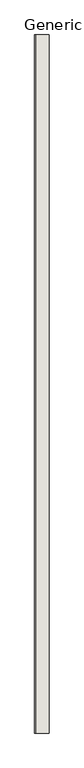
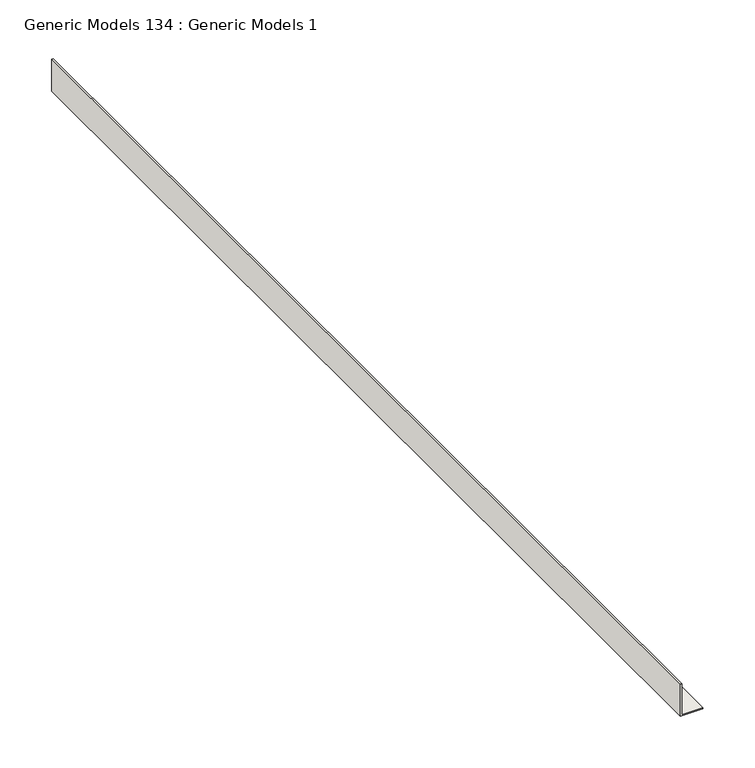
"""IFC4 building model written with IfcOpenShell, lengths in millimetres: wall geometry, Generic Models 134 : Generic Models 1."""

from ifc_helpers import new_model, si_unit, frame, origin, place, context, project, spatial, polyline, outline, extrude, source, transform, mapped, element, save


def generic_models_134_generic_models_1_695f3fb9(model_context):
    return source(origin(), model_context, "Body", "SweptSolid", [
        extrude(outline(polyline([(1860.7484375, 51003.2), (1822.6484375, 51003.2), (1822.6484375, 51028.6), (1824.2359375, 51028.6), (1824.2359375, 51004.7875), (1860.7484375, 51004.7875), (1860.7484375, 51003.2)])), frame((0.0, 0.0, 0.0), z_axis=(0.0, 1.0, 0.0), x_axis=(0.0, 0.0, 1.0)), (0.0, 0.0, 1.0), 1219.2),
    ])


if __name__ == "__main__":
    model = new_model("IFC4")
    model_context = context("Model", 3, world=origin())
    ifc_project = project(units=[si_unit("LENGTHUNIT", "METRE", prefix="MILLI")], contexts=[model_context])
    site = spatial("IfcSite", under=ifc_project)
    building = spatial("IfcBuilding", under=site)
    placement = place(None, origin())
    generic_models_134_generic_models_1_shape = generic_models_134_generic_models_1_695f3fb9(model_context)
    element("IfcWall", 1, ObjectType="Generic Models 134 : Generic Models 1", at=placement, inside=building, context=model_context, shape_type="MappedRepresentation", body=[
        mapped(generic_models_134_generic_models_1_shape, transform((0.0, 0.0, 0.0), x_axis=(1.0, 0.0, 0.0), y_axis=(0.0, 1.0, 0.0), z_axis=(0.0, 0.0, 1.0))),
    ])
    save(model, "model.ifc")

# Revit data of these elements
# Element 1 (IfcWall, "Generic Models 134 : Generic Models 1")
#   Materials on its faces: "CEILING TRACK TO MATCH EXISTING"
# Materials
#   "CEILING TRACK TO MATCH EXISTING": class "Unassigned", colour RGB 210 209 208, transparency 0, Keynote = "M05121300.02", Cost = 0
